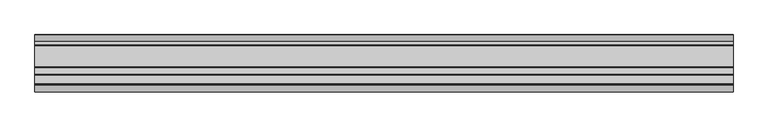
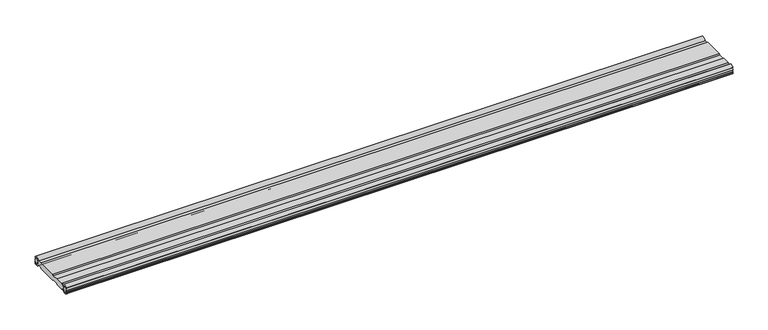
"""IFC4 building model written with IfcOpenShell, lengths in millimetres: proxy geometry, TN_ПВХ_ТПО_Гидрошпонка ТехноНИКОЛЬ : ПВХ Гидрошпонка ТехноНИКОЛЬ IC-125-2SP."""

from ifc_helpers import new_model, si_unit, point, frame, frame_2d, origin, place, context, project, spatial, polyline, circle_curve, trimmed, segment, composite_curve, outline, extrude, source, transform, mapped, element, save


def specialty_equipment_ec462674(model_context):
    return source(origin(), model_context, "Body", "SweptSolid", [
        extrude(outline(composite_curve([segment(trimmed(circle_curve(frame_2d((55.0, 6.8761156)), 8.124571), [point((47.5, 10.0))], [point((61.3988303, 11.882474))], False, "CARTESIAN"), True, "CONTINUOUS"), segment(polyline([(61.3988303, 11.882474), (59.9937159, 10.4773596)]), True, "CONTINUOUS"), segment(trimmed(circle_curve(frame_2d((55.5354706, 5.0)), 7.0623947), [point((59.9937159, 10.4773596))], [point((60.5231974, 0.0))], True, "CARTESIAN"), True, "CONTINUOUS"), segment(polyline([(60.5231974, 0.0), (61.8493138, -1.3261164)]), True, "CONTINUOUS"), segment(trimmed(circle_curve(frame_2d((55.0, 3.0237492)), 8.1138419), [point((61.8493138, -1.3261164))], [point((47.4706328, 0.0))], False, "CARTESIAN"), True, "CONTINUOUS"), segment(polyline([(47.4706328, 0.0), (39.3047128, 0.0), (37.153946, -2.1507668), (-7.846054, -2.1507668), (-9.9968208, 0.0), (-23.2958626, 0.0), (-25.4466295, -2.1507668), (-43.663514, -2.1507668), (-45.8142808, 0.0), (-47.4706328, 0.0)]), True, "CONTINUOUS"), segment(trimmed(circle_curve(frame_2d((-55.0, 3.0237492)), 8.1138419), [point((-47.4706328, 0.0))], [point((-61.8493138, -1.3261164))], False, "CARTESIAN"), True, "CONTINUOUS"), segment(polyline([(-61.8493138, -1.3261164), (-60.5231974, 0.0)]), True, "CONTINUOUS"), segment(trimmed(circle_curve(frame_2d((-55.5354706, 5.0)), 7.0623947), [point((-60.5231974, 0.0))], [point((-59.9937159, 10.4773596))], True, "CARTESIAN"), True, "CONTINUOUS"), segment(polyline([(-59.9937159, 10.4773596), (-61.3988303, 11.882474)]), True, "CONTINUOUS"), segment(trimmed(circle_curve(frame_2d((-55.0, 6.8761156)), 8.124571), [point((-61.3988303, 11.882474))], [point((-47.5, 10.0))], False, "CARTESIAN"), True, "CONTINUOUS"), segment(polyline([(-47.5, 10.0), (-45.8142808, 10.0), (-43.663514, 12.1507668), (-25.4466295, 12.1507668), (-23.2958626, 10.0), (-9.9968208, 10.0), (-7.846054, 12.1507668), (37.153946, 12.1507668), (39.3047128, 10.0), (47.5, 10.0)]), True, "CONTINUOUS")], self_intersect=False)), frame((0.0, 0.0, 0.0), z_axis=(1.0, 0.0, 0.0), x_axis=(0.0, 1.0, 0.0)), (0.0, 0.0, 1.0), 1500.0),
        extrude(outline(composite_curve([segment(trimmed(circle_curve(frame_2d((55.5354706, 5.0)), 5.5168896), [point((50.018581, 5.0))], [point((61.0523602, 5.0))], False, "CARTESIAN"), True, "CONTINUOUS"), segment(trimmed(circle_curve(frame_2d((55.5354706, 5.0)), 5.5168896), [point((61.0523602, 5.0))], [point((50.018581, 5.0))], False, "CARTESIAN"), True, "CONTINUOUS")], self_intersect=False)), frame((0.0, 0.0, 0.0), z_axis=(1.0, 0.0, 0.0), x_axis=(0.0, 1.0, 0.0)), (0.0, 0.0, 1.0), 1500.0),
        extrude(outline(composite_curve([segment(trimmed(circle_curve(frame_2d((-55.5354706, 5.0)), 5.5168896), [point((-50.018581, 5.0))], [point((-61.0523602, 5.0))], False, "CARTESIAN"), True, "CONTINUOUS"), segment(trimmed(circle_curve(frame_2d((-55.5354706, 5.0)), 5.5168896), [point((-61.0523602, 5.0))], [point((-50.018581, 5.0))], False, "CARTESIAN"), True, "CONTINUOUS")], self_intersect=False)), frame((0.0, 0.0, 0.0), z_axis=(1.0, 0.0, 0.0), x_axis=(0.0, 1.0, 0.0)), (0.0, 0.0, 1.0), 1500.0),
    ])


if __name__ == "__main__":
    model = new_model("IFC4")
    model_context = context("Model", 3, world=origin())
    ifc_project = project(units=[si_unit("LENGTHUNIT", "METRE", prefix="MILLI")], contexts=[model_context])
    site = spatial("IfcSite", under=ifc_project)
    building = spatial("IfcBuilding", under=site)
    placement = place(None, origin())
    specialty_equipment_shape = specialty_equipment_ec462674(model_context)
    element("IfcBuildingElementProxy", 1, Name="TN_ПВХ_ТПО_Гидрошпонка ТехноНИКОЛЬ : ПВХ Гидрошпонка ТехноНИКОЛЬ IC-125-2SP", ObjectType="TN_ПВХ_ТПО_Гидрошпонка ТехноНИКОЛЬ : ПВХ Гидрошпонка ТехноНИКОЛЬ IC-125-2SP", at=placement, inside=building, context=model_context, shape_type="MappedRepresentation", body=[
        mapped(specialty_equipment_shape, transform((0.0, 0.0, 0.0), x_axis=(1.0, 0.0, 0.0), y_axis=(0.0, 1.0, 0.0), z_axis=(0.0, 0.0, 1.0))),
    ])
    save(model, "model.ifc")

# Revit data of these elements
# Type "TN_ПВХ_ТПО_Гидрошпонка ТехноНИКОЛЬ : ПВХ Гидрошпонка ТехноНИКОЛЬ IC-125-2SP"
#   Description = "Внутренняя гидрошпонка для герметизации рабочих швов бетонирования в месте сопряжения фундаментной плиты и фундаментных стен в монолитных конструкциях при новом строительстве. Вдоль обоих краев шпонки расположены полимерные набухающие шнуры, которые при контакте с водой увеличиваются в объеме до 350%, обеспечивая дополнительную преграду для проникновения воды. Поставляется в комплекте с металлическими держателями из расчёта 3 шт./п.м."
#   Type Comments = "п.м."
#   Manufacturer = "ТехноНИКОЛЬ"
#   URL = "https://www.tstn.ru/product/pvkh-gidroshponka-tekhnonikol-ic-125-2sp-20-m-rul-644135/"
#   ADSK_Примечание = ""
#   ADSK_Обозначение [instance default] = "ТехноНИКОЛЬ"
#   ADSK_Наименование = "ПВХ Гидрошпонка ТехноНИКОЛЬ IC-125-2SP"
#   ADSK_Масса_Текст = ""
#   ADSK_Марка = ""
#   ADSK_Код изделия = "644135"
#   ADSK_Завод-изготовитель [instance default] = "ТехноНИКОЛЬ"
#   ADSK_Единица измерения [instance default] = "п.м."
#   ADSK_Группирование = "Гидрошпонки"
#   ADSK_URL страницы изделия = "https://www.tstn.ru/product/pvkh-gidroshponka-tekhnonikol-ic-125-2sp-20-m-rul-644135/"
#   ADSK_URL документации изделия = "https://nav.tn.ru/upload/iblock/67f/Katalog-i-rekomendatsii-po-primeneniyu_Gidroshponki-TEKHNONIKOL.PDF"
#   built-in parameter 1001306 [instance default] = 3.28084 (stored number, unit not read)
#   ADSK_Размер_Длина [instance default] = 1000 mm
#   ADSK_Количество [instance default] = 1
#   ПВХ_ТПО Гидрошпонка ТехноНИКОЛЬ EC-320-4 = no
#   ПВХ Гидрошпонка ТехноНИКОЛЬ IM-260/50 = no
#   ПВХ Гидрошпонка ТехноНИКОЛЬ IM-240/20 = no
#   ПВХ Гидрошпонка ТехноНИКОЛЬ IC-240-6 = no
#   ПВХ Гидрошпонка ТехноНИКОЛЬ IC-125-2SP = yes
#   ПВХ Гидрошпонка ТехноНИКОЛЬ EM-260/50 = no
#   ПВХ Гидрошпонка ТехноНИКОЛЬ EM-260/20 = no
#   ПВХ Гидрошпонка ТехноНИКОЛЬ EC-320-4 = no
#   ПВХ Гидрошпонка ТехноНИКОЛЬ EC-220-3 = no
#   ПВХ_ТПО Гидрошпонка ТехноНИКОЛЬ EC-220-3 = no
#   ПВХ Гидрошпонка ТехноНИКОЛЬ IC-240-2 = no
#   Материал = TN_ПВХ_Черный
#   Default Elevation = 0
# Element 1 (IfcBuildingElementProxy, "TN_ПВХ_ТПО_Гидрошпонка ТехноНИКОЛЬ : ПВХ Гидрошпонка ТехноНИКОЛЬ IC-125-2SP")
#   built-in parameter 1001306 = 4.92126 (stored number, unit not read)
#   ADSK_Размер_Длина = 1500 mm
#   ADSK_Количество = 1.5
#   Materials on its faces: "TN_ПВХ_Черный"
# Materials
#   "TN_ПВХ_Черный": class "Типовые", colour RGB 48 48 48, transparency 0, Cost = 0
